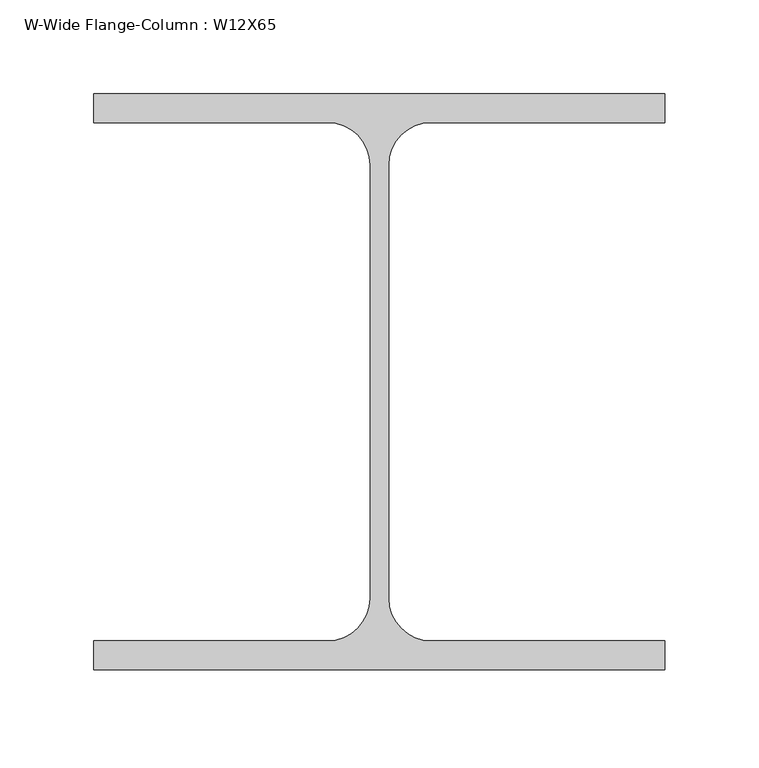
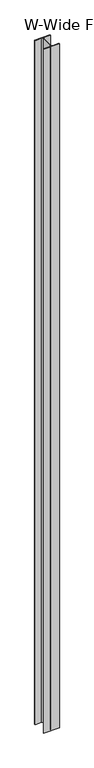
"""IFC4 building model written with IfcOpenShell, lengths in millimetres: column geometry, W-Wide Flange-Column : W12X65."""

import ifcopenshell
import ifcopenshell.guid

model = None  # the IFC model being written
_history = None  # IfcOwnerHistory: only IFC2X3 demands one
_inside = {}  # id of a spatial element -> (the spatial element, [elements in it])
_under = {}  # id of a project, library or spatial element -> (it, [spatial elements below it])
_declared = {}  # id of a project -> (the project, [libraries it declares])
_typed = {}  # id of a type object -> (the type object, [elements of that type])
_made_of = {}  # id of a material, layer set ... -> (it, [elements and type objects made of it])


def new_model(schema):
    """Start an empty IFC model of exactly this schema.

    Asked for "IFC4X3", IfcOpenShell would pick the latest addendum, in which some entities
    have other attributes; the version numbers below select the first issue.
    IFC2X3 requires an IfcOwnerHistory on every rooted entity: one is made here for all.
    """
    global model, _history
    if schema == "IFC4X3":
        model = ifcopenshell.file(schema_version=(4, 3, 0, 0))
    else:
        model = ifcopenshell.file(schema=schema)
    _inside.clear()
    _under.clear()
    _declared.clear()
    _typed.clear()
    _made_of.clear()
    _history = None
    if model.schema == "IFC2X3":
        org = make("IfcOrganization", Name="unknown")
        user = make(
            "IfcPersonAndOrganization",
            ThePerson=make("IfcPerson", FamilyName="unknown"),
            TheOrganization=org,
        )
        app = make(
            "IfcApplication",
            ApplicationDeveloper=org,
            Version="unknown",
            ApplicationFullName="unknown",
            ApplicationIdentifier="unknown",
        )
        _history = make(
            "IfcOwnerHistory",
            OwningUser=user,
            OwningApplication=app,
            ChangeAction="ADDED",
            CreationDate=0,
        )
    return model


def make(cls, **values):
    """One entity of the class cls with the attributes given. An attribute that is None is left unset."""
    return model.create_entity(
        cls, **{name: value for name, value in values.items() if value is not None}
    )


def rooted(cls, **values):
    """An entity with a GlobalId (a new one), such as an element, a storey or a relation."""
    return make(cls, GlobalId=ifcopenshell.guid.new(), OwnerHistory=_history, **values)


def si_unit(unit_type, name, prefix=None):
    """IfcSIUnit, for example si_unit("LENGTHUNIT", "METRE", prefix="MILLI")."""
    return make("IfcSIUnit", UnitType=unit_type, Prefix=prefix, Name=name)


def assignment(units):
    """IfcUnitAssignment: the units of a project."""
    return None if units is None else make("IfcUnitAssignment", Units=units)


def point(xyz):
    """IfcCartesianPoint."""
    return None if xyz is None else make("IfcCartesianPoint", Coordinates=xyz)


def direction(xyz):
    """IfcDirection."""
    return None if xyz is None else make("IfcDirection", DirectionRatios=xyz)


def frame(location, z_axis=None, x_axis=None):
    """IfcAxis2Placement3D, a coordinate frame: its origin and axes. An axis left out is left unset."""
    return make(
        "IfcAxis2Placement3D",
        Location=point(location),
        Axis=direction(z_axis),
        RefDirection=direction(x_axis),
    )


def frame_2d(location, x_axis=None):
    """IfcAxis2Placement2D, a coordinate frame in the plane: its origin and x axis."""
    return make(
        "IfcAxis2Placement2D", Location=point(location), RefDirection=direction(x_axis)
    )


def origin():
    """The frame at (0, 0, 0) with its axes left unset."""
    return frame((0.0, 0.0, 0.0))


def place(relative_to, where):
    """IfcLocalPlacement: puts the frame where relative to a parent placement (None: the world)."""
    return make(
        "IfcLocalPlacement", PlacementRelTo=relative_to, RelativePlacement=where
    )


def context(
    kind, dimensions, precision=None, world=None, true_north=None, identifier=None
):
    """IfcGeometricRepresentationContext, for example the 3D "Model" context."""
    return make(
        "IfcGeometricRepresentationContext",
        ContextIdentifier=identifier,
        ContextType=kind,
        CoordinateSpaceDimension=dimensions,
        Precision=precision,
        WorldCoordinateSystem=world,
        TrueNorth=true_north,
    )


def project(units=None, contexts=None):
    """IfcProject with its units and contexts."""
    return rooted(
        "IfcProject",
        Name="project",
        RepresentationContexts=contexts,
        UnitsInContext=assignment(units),
    )


def spatial(cls, under=None, at=None, **own):
    """A site, building, storey or space (cls), placed at a placement, below another one or the project."""
    s = rooted(cls, ObjectPlacement=at, **own)
    if under is not None:
        _under.setdefault(under.id(), (under, []))[1].append(s)
    return s


def polyline(points):
    """IfcPolyline through the points."""
    return make("IfcPolyline", Points=[point(p) for p in points])


def circle_curve(where, radius):
    """IfcCircle in the frame where."""
    return make("IfcCircle", Position=where, Radius=radius)


def trimmed(basis, trim1, trim2, sense, master):
    """IfcTrimmedCurve: the piece of a basis curve between two trims."""
    return make(
        "IfcTrimmedCurve",
        BasisCurve=basis,
        Trim1=trim1,
        Trim2=trim2,
        SenseAgreement=sense,
        MasterRepresentation=master,
    )


def segment(curve, same_sense, transition):
    """IfcCompositeCurveSegment."""
    return make(
        "IfcCompositeCurveSegment",
        Transition=transition,
        SameSense=same_sense,
        ParentCurve=curve,
    )


def composite_curve(segments, self_intersect=None):
    """IfcCompositeCurve: segments joined end to end."""
    return make("IfcCompositeCurve", Segments=segments, SelfIntersect=self_intersect)


def outline(outer, holes=None, kind="AREA"):
    """IfcArbitraryClosedProfileDef: a profile drawn as a closed curve; with holes, ...WithVoids."""
    if holes is None:
        return make("IfcArbitraryClosedProfileDef", ProfileType=kind, OuterCurve=outer)
    return make(
        "IfcArbitraryProfileDefWithVoids",
        ProfileType=kind,
        OuterCurve=outer,
        InnerCurves=holes,
    )


def extrude(swept, where, along, depth):
    """IfcExtrudedAreaSolid: the profile swept, set in the frame where, extruded along a direction by depth."""
    return make(
        "IfcExtrudedAreaSolid",
        SweptArea=swept,
        Position=where,
        ExtrudedDirection=direction(along),
        Depth=depth,
    )


def shape(context_of_items, identifier, shape_type, items):
    """IfcShapeRepresentation: the items that make up one representation, for example the "Body"."""
    return make(
        "IfcShapeRepresentation",
        ContextOfItems=context_of_items,
        RepresentationIdentifier=identifier,
        RepresentationType=shape_type,
        Items=items,
    )


def source(mapping_origin, context_of_items, identifier, shape_type, items):
    """IfcRepresentationMap: a shape defined once, which mapped items show again and again."""
    return make(
        "IfcRepresentationMap",
        MappingOrigin=mapping_origin,
        MappedRepresentation=shape(context_of_items, identifier, shape_type, items),
    )


def transform(
    local_origin,
    x_axis=None,
    y_axis=None,
    z_axis=None,
    scale=None,
    scale2=None,
    scale3=None,
    uniform=True,
):
    """IfcCartesianTransformationOperator3D, or its non-uniform kind. x_axis, y_axis, z_axis: its Axis1, 2, 3."""
    if uniform:
        return make(
            "IfcCartesianTransformationOperator3D",
            Axis1=direction(x_axis),
            Axis2=direction(y_axis),
            LocalOrigin=point(local_origin),
            Scale=scale,
            Axis3=direction(z_axis),
        )
    return make(
        "IfcCartesianTransformationOperator3DnonUniform",
        Axis1=direction(x_axis),
        Axis2=direction(y_axis),
        LocalOrigin=point(local_origin),
        Scale=scale,
        Axis3=direction(z_axis),
        Scale2=scale2,
        Scale3=scale3,
    )


def mapped(mapping_source, mapping_target):
    """IfcMappedItem: shows the shape of a source again, moved by a transform."""
    return make(
        "IfcMappedItem", MappingSource=mapping_source, MappingTarget=mapping_target
    )


def made_of(thing, what):
    """Note that an element or type object is made of a material, layer set ...; save() writes the relation."""
    if what is not None:
        _made_of.setdefault(what.id(), (what, []))[1].append(thing)
    return thing


def element(
    cls,
    number,
    at=None,
    inside=None,
    cuts=None,
    type_object=None,
    material=None,
    context=None,
    identifier="Body",
    shape_type=None,
    held_by="IfcProductDefinitionShape",
    body=None,
    shapes=None,
    **own,
):
    """One element of the class cls, such as IfcWall. Its Tag is "e" and its number.

    at: its placement. inside: the storey or other place that contains it. cuts: it is an
    opening in that element (IfcRelVoidsElement). A single representation is given by context,
    identifier, shape_type and body (its items); several are given by shapes. held_by: the class
    of the entity that holds the representations. save() writes the other relations.
    """
    e = rooted(cls, Tag="e%d" % number, ObjectPlacement=at, **own)
    if body is not None:
        shapes = [shape(context, identifier, shape_type, body)]
    if shapes is not None:
        e.Representation = make(held_by, Representations=shapes)
    if inside is not None:
        _inside.setdefault(inside.id(), (inside, []))[1].append(e)
    if cuts is not None:
        rooted(
            "IfcRelVoidsElement", RelatingBuildingElement=cuts, RelatedOpeningElement=e
        )
    if type_object is not None:
        _typed.setdefault(type_object.id(), (type_object, []))[1].append(e)
    return made_of(e, material)


def aggregate(whole, parts):
    """IfcRelAggregates: a whole, such as a stair, and the parts it consists of."""
    return rooted("IfcRelAggregates", RelatingObject=whole, RelatedObjects=parts)


def save(model, path):
    """Write the relations noted so far, then the file.

    IfcRelAggregates (storeys below a building ...), IfcRelContainedInSpatialStructure (elements
    in a storey), IfcRelDefinesByType, IfcRelAssociatesMaterial and IfcRelDeclares: one each for
    every whole, place, type object, material and project.
    """
    for whole, parts in _under.values():
        aggregate(whole, parts)
    for where, things in _inside.values():
        rooted(
            "IfcRelContainedInSpatialStructure",
            RelatedElements=things,
            RelatingStructure=where,
        )
    for kind, things in _typed.values():
        rooted("IfcRelDefinesByType", RelatedObjects=things, RelatingType=kind)
    for what, things in _made_of.values():
        rooted("IfcRelAssociatesMaterial", RelatedObjects=things, RelatingMaterial=what)
    for by, libraries in _declared.values():
        rooted("IfcRelDeclares", RelatingContext=by, RelatedDefinitions=libraries)
    model.write(path)


def w_wide_flange_column_w12x65_25bd69bb(model_context):
    return source(origin(), model_context, "Body", "SweptSolid", [
        extrude(outline(composite_curve([segment(polyline([(152.4, 153.67), (152.4, 138.303), (27.686, 138.303)]), True, "CONTINUOUS"), segment(trimmed(circle_curve(frame_2d((27.686, 115.57)), 22.733), [point((27.686, 138.303))], [point((4.953, 115.57))], True, "CARTESIAN"), True, "CONTINUOUS"), segment(polyline([(4.953, 115.57), (4.953, -115.57)]), True, "CONTINUOUS"), segment(trimmed(circle_curve(frame_2d((27.686, -115.57)), 22.733), [point((4.953, -115.57))], [point((27.686, -138.303))], True, "CARTESIAN"), True, "CONTINUOUS"), segment(polyline([(27.686, -138.303), (152.4, -138.303), (152.4, -153.67), (-152.4, -153.67), (-152.4, -138.303), (-27.686, -138.303)]), True, "CONTINUOUS"), segment(trimmed(circle_curve(frame_2d((-27.686, -115.57)), 22.733), [point((-27.686, -138.303))], [point((-4.953, -115.57))], True, "CARTESIAN"), True, "CONTINUOUS"), segment(polyline([(-4.953, -115.57), (-4.953, 115.57)]), True, "CONTINUOUS"), segment(trimmed(circle_curve(frame_2d((-27.686, 115.57)), 22.733), [point((-4.953, 115.57))], [point((-27.686, 138.303))], True, "CARTESIAN"), True, "CONTINUOUS"), segment(polyline([(-27.686, 138.303), (-152.4, 138.303), (-152.4, 153.67), (152.4, 153.67)]), True, "CONTINUOUS")], self_intersect=False)), frame((0.0, 0.0, 9163.05), z_axis=(0.0, 0.0, 1.0), x_axis=(1.0, 0.0, 0.0)), (0.0, 0.0, 1.0), 14154.15),
    ])


if __name__ == "__main__":
    model = new_model("IFC4")
    model_context = context("Model", 3, world=origin())
    ifc_project = project(units=[si_unit("LENGTHUNIT", "METRE", prefix="MILLI")], contexts=[model_context])
    site = spatial("IfcSite", under=ifc_project)
    building = spatial("IfcBuilding", under=site)
    placement = place(None, origin())
    w_wide_flange_column_w12x65_shape = w_wide_flange_column_w12x65_25bd69bb(model_context)
    element("IfcColumn", 1, ObjectType="W-Wide Flange-Column : W12X65", at=placement, inside=building, context=model_context, shape_type="MappedRepresentation", body=[
        mapped(w_wide_flange_column_w12x65_shape, transform((0.0, 0.0, 0.0), x_axis=(1.0, 0.0, 0.0), y_axis=(0.0, 1.0, 0.0), z_axis=(0.0, 0.0, 1.0))),
    ])
    save(model, "model.ifc")

# Revit data of these elements
# Type "W-Wide Flange-Column : W12X65"
#   Assembly Code = "B10"
#   W = 65
#   bf = 1' - 0"
#   d = 1' - 0.1"
#   k = 0' - 1 1/2"
#   kr = 0' - 0.895"
#   tf = 0' - 0.605"
#   tw = 0' - 0.39"
#   A = 0.132639 SF
#   Structural Material [instance default] = Steel ASTM A992
# Element 1 (IfcColumn, "W-Wide Flange-Column : W12X65")
#   Materials on its faces: "Steel ASTM A992"
# Materials
#   "Steel ASTM A992": class "Metal", colour RGB 199 199 199, transparency 0, Description = "Structural steel 50ksi", Cost = 0
